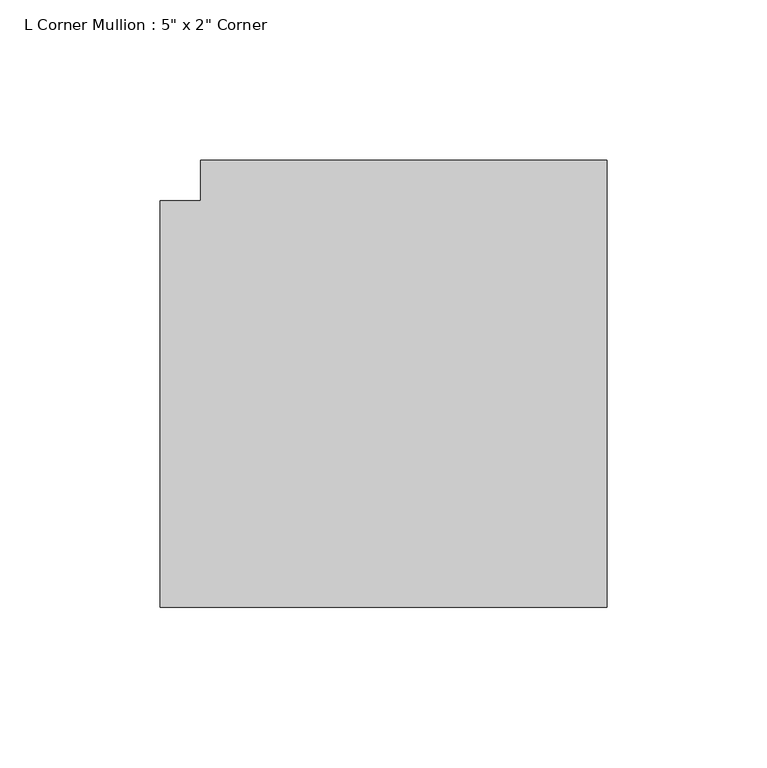
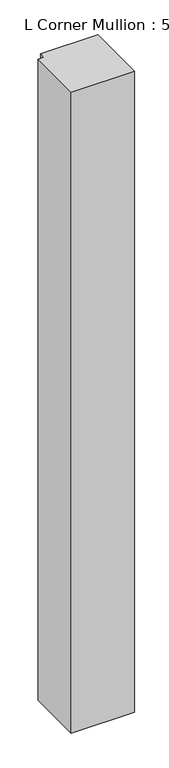
"""IFC4 building model written with IfcOpenShell, lengths in millimetres: member geometry."""

from ifc_helpers import new_model, si_unit, frame, origin, place, context, project, spatial, polyline, outline, extrude, source, transform, mapped, element, save


def member_ad26c05c(model_context):
    return source(origin(), model_context, "Body", "SweptSolid", [
        extrude(outline(polyline([(63.5, 76.2), (63.5, -63.5), (-76.2, -63.5), (-76.2, 63.5), (-63.5, 63.5), (-63.5, 76.2), (63.5, 76.2)])), frame((0.0, 0.0, -1498.6), z_axis=(0.0, 0.0, 1.0), x_axis=(1.0, 0.0, 0.0)), (0.0, 0.0, 1.0), 1498.6),
    ])


if __name__ == "__main__":
    model = new_model("IFC4")
    model_context = context("Model", 3, world=origin())
    ifc_project = project(units=[si_unit("LENGTHUNIT", "METRE", prefix="MILLI")], contexts=[model_context])
    site = spatial("IfcSite", under=ifc_project)
    building = spatial("IfcBuilding", under=site)
    placement = place(None, origin())
    member_shape = member_ad26c05c(model_context)
    element("IfcMember", 1, ObjectType="L Corner Mullion : 5\" x 2\" Corner", at=placement, inside=building, context=model_context, shape_type="MappedRepresentation", body=[
        mapped(member_shape, transform((0.0, 0.0, 0.0), x_axis=(1.0, 0.0, 0.0), y_axis=(0.0, 1.0, 0.0), z_axis=(0.0, 0.0, 1.0))),
    ])
    save(model, "model.ifc")

# Revit data of these elements
# Type "L Corner Mullion : 5\" x 2\" Corner"
#   built-in parameter 1007355 = 0.25 (stored number, unit not read)
#   built-in parameter 1007354 = 0.25 (stored number, unit not read)
#   built-in parameter 1007304 = 0.416667 (stored number, unit not read)
# Element 1 (IfcMember, "L Corner Mullion : 5\" x 2\" Corner")
#   Materials on its faces: "Metal - Aluminum"
# Materials
#   "Metal - Aluminum": class "Metal", colour RGB 109 108 108, transparency 0
